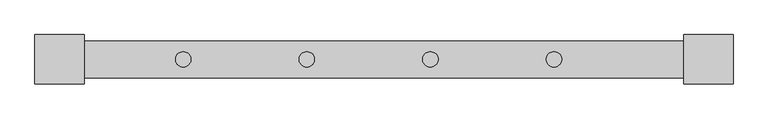
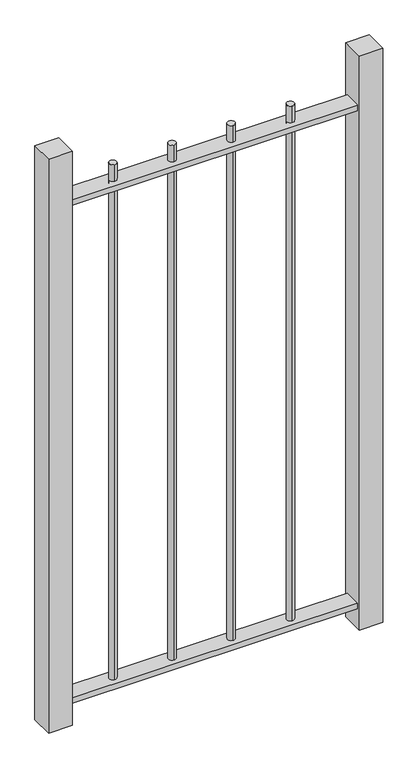
"""IFC4 building model written with IfcOpenShell, lengths in millimetres: railing geometry."""

from ifc_helpers import new_model, si_unit, point, frame, frame_2d, origin, place, context, project, spatial, polyline, circle_curve, trimmed, segment, composite_curve, outline, extrude, source, transform, mapped, element, save


def railing_98353e33(model_context):
    return source(origin(), model_context, "Body", "SweptSolid", [
        extrude(outline(polyline([(-3469.419961, -24961.1119119), (-3469.419961, -24901.1119119), (-2419.419961, -24901.1119119), (-2419.419961, -24961.1119119), (-3469.419961, -24961.1119119)])), frame((0.0, 0.0, -30.0), z_axis=(0.0, 0.0, 1.0), x_axis=(1.0, 0.0, 0.0)), (0.0, 0.0, 1.0), 20.0),
        extrude(outline(polyline([(-3469.419961, -24961.1119119), (-3469.419961, -24901.1119119), (-2419.419961, -24901.1119119), (-2419.419961, -24961.1119119), (-3469.419961, -24961.1119119)])), frame((0.0, 0.0, 1750.0), z_axis=(0.0, 0.0, 1.0), x_axis=(1.0, 0.0, 0.0)), (0.0, 0.0, 1.0), 20.0),
        extrude(outline(composite_curve([segment(trimmed(circle_curve(frame_2d((-2669.419961, -24931.1119119)), 12.5), [point((-2669.419961, -24943.6119119))], [point((-2669.419961, -24918.6119119))], False, "CARTESIAN"), True, "CONTINUOUS"), segment(trimmed(circle_curve(frame_2d((-2669.419961, -24931.1119119)), 12.5), [point((-2669.419961, -24918.6119119))], [point((-2669.419961, -24943.6119119))], False, "CARTESIAN"), True, "CONTINUOUS")], self_intersect=False)), frame((0.0, 0.0, -10.0), z_axis=(0.0, 0.0, 1.0), x_axis=(1.0, 0.0, 0.0)), (0.0, 0.0, 1.0), 1840.0),
        extrude(outline(composite_curve([segment(trimmed(circle_curve(frame_2d((-2869.419961, -24931.1119119)), 12.5), [point((-2869.419961, -24943.6119119))], [point((-2869.419961, -24918.6119119))], False, "CARTESIAN"), True, "CONTINUOUS"), segment(trimmed(circle_curve(frame_2d((-2869.419961, -24931.1119119)), 12.5), [point((-2869.419961, -24918.6119119))], [point((-2869.419961, -24943.6119119))], False, "CARTESIAN"), True, "CONTINUOUS")], self_intersect=False)), frame((0.0, 0.0, -10.0), z_axis=(0.0, 0.0, 1.0), x_axis=(1.0, 0.0, 0.0)), (0.0, 0.0, 1.0), 1840.0),
        extrude(outline(composite_curve([segment(trimmed(circle_curve(frame_2d((-3069.419961, -24931.1119119)), 12.5), [point((-3069.419961, -24943.6119119))], [point((-3069.419961, -24918.6119119))], False, "CARTESIAN"), True, "CONTINUOUS"), segment(trimmed(circle_curve(frame_2d((-3069.419961, -24931.1119119)), 12.5), [point((-3069.419961, -24918.6119119))], [point((-3069.419961, -24943.6119119))], False, "CARTESIAN"), True, "CONTINUOUS")], self_intersect=False)), frame((0.0, 0.0, -10.0), z_axis=(0.0, 0.0, 1.0), x_axis=(1.0, 0.0, 0.0)), (0.0, 0.0, 1.0), 1840.0),
        extrude(outline(composite_curve([segment(trimmed(circle_curve(frame_2d((-3269.419961, -24931.1119119)), 12.5), [point((-3269.419961, -24943.6119119))], [point((-3269.419961, -24918.6119119))], False, "CARTESIAN"), True, "CONTINUOUS"), segment(trimmed(circle_curve(frame_2d((-3269.419961, -24931.1119119)), 12.5), [point((-3269.419961, -24918.6119119))], [point((-3269.419961, -24943.6119119))], False, "CARTESIAN"), True, "CONTINUOUS")], self_intersect=False)), frame((0.0, 0.0, -10.0), z_axis=(0.0, 0.0, 1.0), x_axis=(1.0, 0.0, 0.0)), (0.0, 0.0, 1.0), 1840.0),
        extrude(outline(polyline([(-2459.419961, -24891.1119119), (-2379.419961, -24891.1119119), (-2379.419961, -24971.1119119), (-2459.419961, -24971.1119119), (-2459.419961, -24891.1119119)])), frame((0.0, 0.0, -100.0), z_axis=(0.0, 0.0, 1.0), x_axis=(1.0, 0.0, 0.0)), (0.0, 0.0, 1.0), 2050.0),
        extrude(outline(polyline([(-3509.419961, -24891.1119119), (-3429.419961, -24891.1119119), (-3429.419961, -24971.1119119), (-3509.419961, -24971.1119119), (-3509.419961, -24891.1119119)])), frame((0.0, 0.0, -100.0), z_axis=(0.0, 0.0, 1.0), x_axis=(1.0, 0.0, 0.0)), (0.0, 0.0, 1.0), 2050.0),
    ])


if __name__ == "__main__":
    model = new_model("IFC4")
    model_context = context("Model", 3, world=origin())
    ifc_project = project(units=[si_unit("LENGTHUNIT", "METRE", prefix="MILLI")], contexts=[model_context])
    site = spatial("IfcSite", under=ifc_project)
    building = spatial("IfcBuilding", under=site)
    placement = place(None, origin())
    railing_shape = railing_98353e33(model_context)
    element("IfcRailing", 1, at=placement, inside=building, context=model_context, shape_type="MappedRepresentation", body=[
        mapped(railing_shape, transform((0.0, 0.0, 0.0), x_axis=(1.0, 0.0, 0.0), y_axis=(0.0, 1.0, 0.0), z_axis=(0.0, 0.0, 1.0))),
    ])
    save(model, "model.ifc")

# Revit data of these elements
# Element 1 (IfcRailing)
#   Materials on its faces: "NLRS_h2_staal_generiek zwart_gen_rsf", "NLRS_h2_staal_gen_rsf"
# Materials
#   "NLRS_h2_staal_generiek zwart_gen_rsf": class "Metal", colour RGB 189 187 185, transparency 0, Manufacturer = "RevitGG", URL = "www.revitgg.nl", Description = "Staal, generiek materiaal", Cost = 0
#   "NLRS_h2_staal_gen_rsf": class "H - Metaal", colour RGB 189 187 185, transparency 0, Keynote = "h2", Model = "generiek", Manufacturer = "Revit Standards Foundation", URL = "www.revitstandards.org", Description = "staal", Cost = 0
